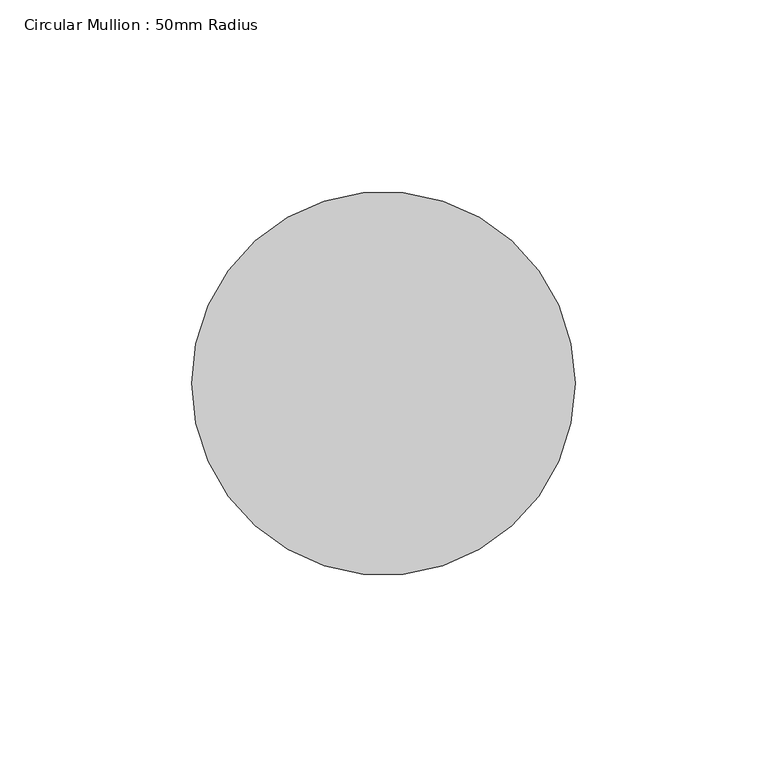
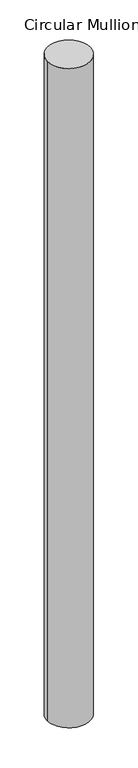
"""IFC4 building model written with IfcOpenShell, lengths in millimetres: member geometry, Circular Mullion : 50mm Radius."""

from ifc_helpers import new_model, si_unit, point, frame, origin, origin_2d, place, context, project, spatial, circle_curve, trimmed, segment, composite_curve, outline, extrude, source, transform, mapped, element, save


def circular_mullion_50mm_radius_f37aa788(model_context):
    return source(origin(), model_context, "Body", "SweptSolid", [
        extrude(outline(composite_curve([segment(trimmed(circle_curve(origin_2d(), 50.0), [point((50.0, 0.0))], [point((-50.0, 0.0))], False, "CARTESIAN"), True, "CONTINUOUS"), segment(trimmed(circle_curve(origin_2d(), 50.0), [point((-50.0, 0.0))], [point((50.0, 0.0))], False, "CARTESIAN"), True, "CONTINUOUS")], self_intersect=False)), frame((0.0, 0.0, -1624.3772675), z_axis=(0.0, 0.0, 1.0), x_axis=(1.0, 0.0, 0.0)), (0.0, 0.0, 1.0), 1624.3772675),
    ])


if __name__ == "__main__":
    model = new_model("IFC4")
    model_context = context("Model", 3, world=origin())
    ifc_project = project(units=[si_unit("LENGTHUNIT", "METRE", prefix="MILLI")], contexts=[model_context])
    site = spatial("IfcSite", under=ifc_project)
    building = spatial("IfcBuilding", under=site)
    placement = place(None, origin())
    circular_mullion_50mm_radius_shape = circular_mullion_50mm_radius_f37aa788(model_context)
    element("IfcMember", 1, ObjectType="Circular Mullion : 50mm Radius", at=placement, inside=building, context=model_context, shape_type="MappedRepresentation", body=[
        mapped(circular_mullion_50mm_radius_shape, transform((0.0, 0.0, 0.0), x_axis=(1.0, 0.0, 0.0), y_axis=(0.0, 1.0, 0.0), z_axis=(0.0, 0.0, 1.0))),
    ])
    save(model, "model.ifc")

# Revit data of these elements
# Type "Circular Mullion : 50mm Radius"
#   built-in parameter 1007350 = 0.164042 (stored number, unit not read)
# Element 1 (IfcMember, "Circular Mullion : 50mm Radius")
#   Materials on its faces: "Aluminium"
# Materials
#   "Aluminium": class "Metal", colour RGB 247 247 247, transparency 0, Description = "Aluminium 6061", Cost = 0
